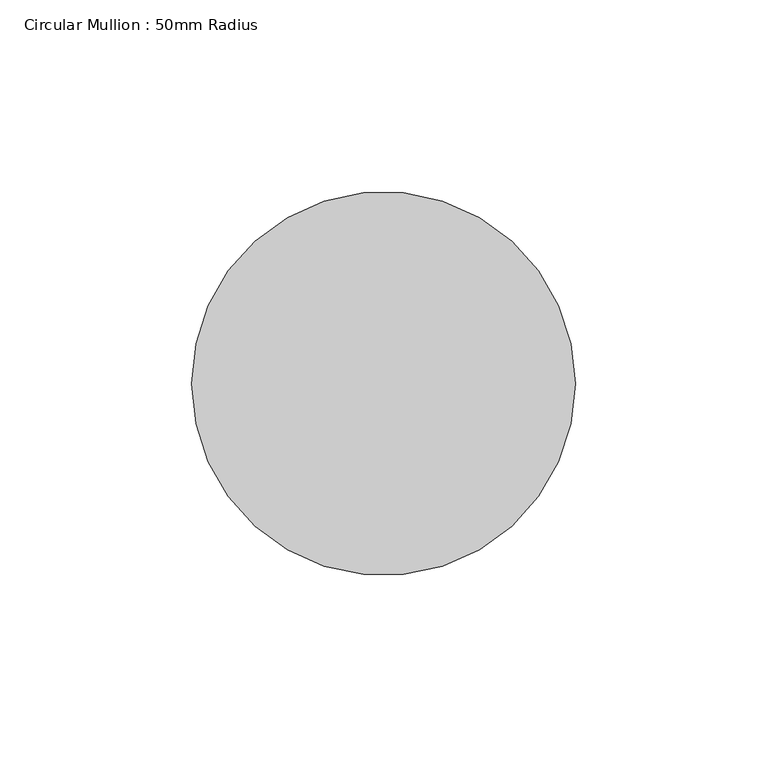
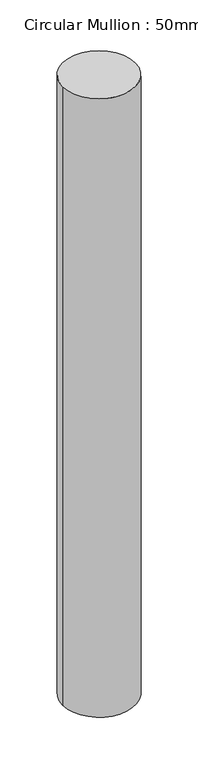
"""IFC4 building model written with IfcOpenShell, lengths in millimetres: member geometry, Circular Mullion : 50mm Radius."""

from ifc_helpers import new_model, si_unit, point, frame, origin, origin_2d, place, context, project, spatial, circle_curve, trimmed, segment, composite_curve, outline, extrude, source, transform, mapped, element, save


def circular_mullion_50mm_radius_05fab217(model_context):
    return source(origin(), model_context, "Body", "SweptSolid", [
        extrude(outline(composite_curve([segment(trimmed(circle_curve(origin_2d(), 50.0), [point((50.0, 0.0))], [point((-50.0, 0.0))], False, "CARTESIAN"), True, "CONTINUOUS"), segment(trimmed(circle_curve(origin_2d(), 50.0), [point((-50.0, 0.0))], [point((50.0, 0.0))], False, "CARTESIAN"), True, "CONTINUOUS")], self_intersect=False)), frame((0.0, 0.0, -900.5124066), z_axis=(0.0, 0.0, 1.0), x_axis=(1.0, 0.0, 0.0)), (0.0, 0.0, 1.0), 900.5124066),
    ])


if __name__ == "__main__":
    model = new_model("IFC4")
    model_context = context("Model", 3, world=origin())
    ifc_project = project(units=[si_unit("LENGTHUNIT", "METRE", prefix="MILLI")], contexts=[model_context])
    site = spatial("IfcSite", under=ifc_project)
    building = spatial("IfcBuilding", under=site)
    placement = place(None, origin())
    circular_mullion_50mm_radius_shape = circular_mullion_50mm_radius_05fab217(model_context)
    element("IfcMember", 1, ObjectType="Circular Mullion : 50mm Radius", at=placement, inside=building, context=model_context, shape_type="MappedRepresentation", body=[
        mapped(circular_mullion_50mm_radius_shape, transform((0.0, 0.0, 0.0), x_axis=(1.0, 0.0, 0.0), y_axis=(0.0, 1.0, 0.0), z_axis=(0.0, 0.0, 1.0))),
    ])
    save(model, "model.ifc")

# Revit data of these elements
# Type "Circular Mullion : 50mm Radius"
#   built-in parameter 1007350 = 0.164042 (stored number, unit not read)
# Element 1 (IfcMember, "Circular Mullion : 50mm Radius")
#   Materials on its faces: "Aluminium"
# Materials
#   "Aluminium": class "Metal", colour RGB 247 247 247, transparency 0, Description = "Aluminium 6061", Cost = 0
